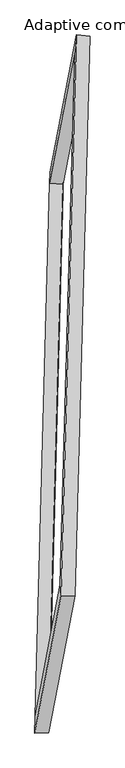
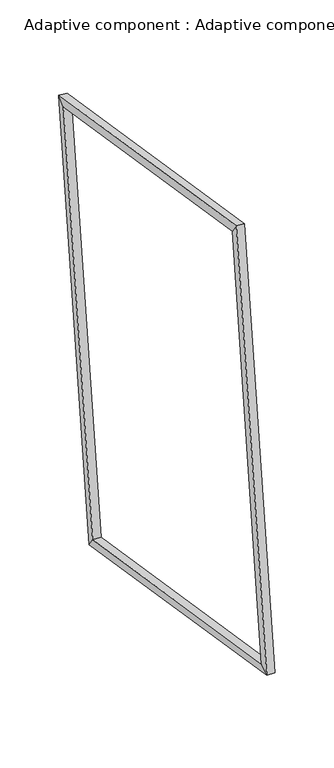
"""IFC4 building model written with IfcOpenShell, lengths in millimetres: proxy geometry, Adaptive component : Adaptive component."""

from ifc_helpers import new_model, si_unit, origin, place, context, project, spatial, faceted_brep, source, transform, mapped, element, save


def adaptive_component_adaptive_component_535112df(model_context):
    return source(origin(), model_context, "Body", "Brep", [
        faceted_brep([(70.4640218, 1145.2617046, 2766.7525641), (135.1152661, 1139.3241131, 2762.212345), (67.0483336, -1361.8424987, 3233.6510735), (2.2225865, -1362.3171337, 3239.3999173), (77.7589774, 1220.8830013, 2818.4009052), (6.0465576, -1414.2395683, 3315.088662), (142.4102216, 1214.9454098, 2813.8606861), (70.8723046, -1413.7649333, 3309.3398181), (-52.180503, -1981.9379759, -73.4120733), (-117.2374075, -1983.614834, -74.0748672), (-118.0113211, -2059.4503379, -125.9181449), (-52.9544166, -2057.7734798, -125.255351), (15.8864295, 519.2286359, -544.8508018), (-48.9959722, 523.9640043, -546.7222205), (-46.2989013, 575.6722317, -622.6059016), (18.5835004, 570.9368633, -620.7344829)], [[[0, 1, 2, 3]], [[4, 0, 3, 5]], [[6, 4, 5, 7]], [[1, 6, 7, 2]], [[3, 2, 8, 9]], [[5, 3, 9, 10]], [[7, 5, 10, 11]], [[2, 7, 11, 8]], [[9, 8, 12, 13]], [[10, 9, 13, 14]], [[11, 10, 14, 15]], [[8, 11, 15, 12]], [[13, 12, 1, 0]], [[14, 13, 0, 4]], [[15, 14, 4, 6]], [[12, 15, 6, 1]]]),
    ])


if __name__ == "__main__":
    model = new_model("IFC4")
    model_context = context("Model", 3, world=origin())
    ifc_project = project(units=[si_unit("LENGTHUNIT", "METRE", prefix="MILLI")], contexts=[model_context])
    site = spatial("IfcSite", under=ifc_project)
    building = spatial("IfcBuilding", under=site)
    placement = place(None, origin())
    adaptive_component_adaptive_component_shape = adaptive_component_adaptive_component_535112df(model_context)
    element("IfcBuildingElementProxy", 1, Name="Adaptive component : Adaptive component", ObjectType="Adaptive component : Adaptive component", at=placement, inside=building, context=model_context, shape_type="MappedRepresentation", body=[
        mapped(adaptive_component_adaptive_component_shape, transform((0.0, 0.0, 0.0), x_axis=(1.0, 0.0, 0.0), y_axis=(0.0, 1.0, 0.0), z_axis=(0.0, 0.0, 1.0))),
    ])
    save(model, "model.ifc")

# Revit data of these elements
# Type "Adaptive component : Adaptive component"
#   r [instance default] = 2063.125 mm
#   2r [instance default] = 4126.251 mm
#   Number [instance default] = 5
#   Default Elevation = 0
# Element 1 (IfcBuildingElementProxy, "Adaptive component : Adaptive component")
#   r = 2203.9 mm
#   2r = 4407.8 mm
#   Number = 10
